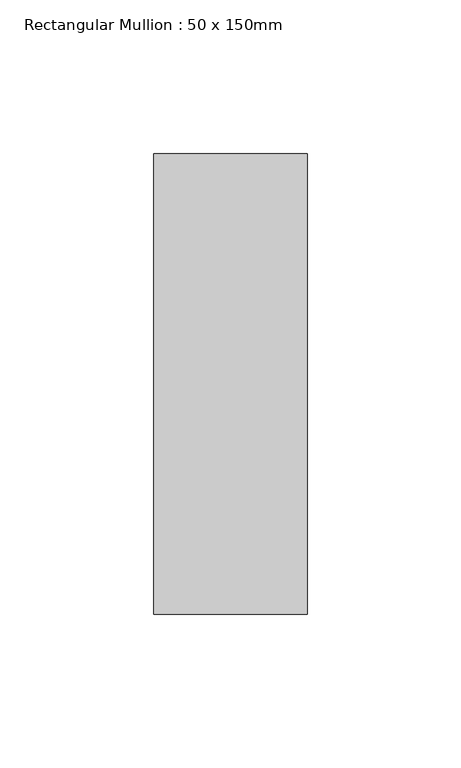
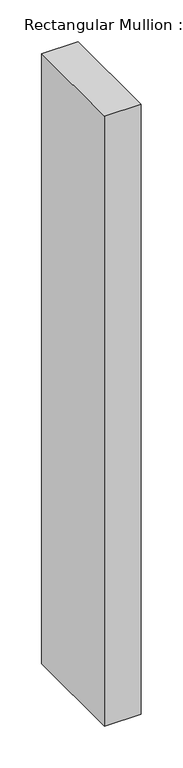
"""IFC4 building model written with IfcOpenShell, lengths in millimetres: member geometry, Rectangular Mullion : 50 x 150mm."""

import ifcopenshell
import ifcopenshell.guid

model = None  # the IFC model being written
_history = None  # IfcOwnerHistory: only IFC2X3 demands one
_inside = {}  # id of a spatial element -> (the spatial element, [elements in it])
_under = {}  # id of a project, library or spatial element -> (it, [spatial elements below it])
_declared = {}  # id of a project -> (the project, [libraries it declares])
_typed = {}  # id of a type object -> (the type object, [elements of that type])
_made_of = {}  # id of a material, layer set ... -> (it, [elements and type objects made of it])


def new_model(schema):
    """Start an empty IFC model of exactly this schema.

    Asked for "IFC4X3", IfcOpenShell would pick the latest addendum, in which some entities
    have other attributes; the version numbers below select the first issue.
    IFC2X3 requires an IfcOwnerHistory on every rooted entity: one is made here for all.
    """
    global model, _history
    if schema == "IFC4X3":
        model = ifcopenshell.file(schema_version=(4, 3, 0, 0))
    else:
        model = ifcopenshell.file(schema=schema)
    _inside.clear()
    _under.clear()
    _declared.clear()
    _typed.clear()
    _made_of.clear()
    _history = None
    if model.schema == "IFC2X3":
        org = make("IfcOrganization", Name="unknown")
        user = make(
            "IfcPersonAndOrganization",
            ThePerson=make("IfcPerson", FamilyName="unknown"),
            TheOrganization=org,
        )
        app = make(
            "IfcApplication",
            ApplicationDeveloper=org,
            Version="unknown",
            ApplicationFullName="unknown",
            ApplicationIdentifier="unknown",
        )
        _history = make(
            "IfcOwnerHistory",
            OwningUser=user,
            OwningApplication=app,
            ChangeAction="ADDED",
            CreationDate=0,
        )
    return model


def make(cls, **values):
    """One entity of the class cls with the attributes given. An attribute that is None is left unset."""
    return model.create_entity(
        cls, **{name: value for name, value in values.items() if value is not None}
    )


def rooted(cls, **values):
    """An entity with a GlobalId (a new one), such as an element, a storey or a relation."""
    return make(cls, GlobalId=ifcopenshell.guid.new(), OwnerHistory=_history, **values)


def si_unit(unit_type, name, prefix=None):
    """IfcSIUnit, for example si_unit("LENGTHUNIT", "METRE", prefix="MILLI")."""
    return make("IfcSIUnit", UnitType=unit_type, Prefix=prefix, Name=name)


def assignment(units):
    """IfcUnitAssignment: the units of a project."""
    return None if units is None else make("IfcUnitAssignment", Units=units)


def point(xyz):
    """IfcCartesianPoint."""
    return None if xyz is None else make("IfcCartesianPoint", Coordinates=xyz)


def direction(xyz):
    """IfcDirection."""
    return None if xyz is None else make("IfcDirection", DirectionRatios=xyz)


def frame(location, z_axis=None, x_axis=None):
    """IfcAxis2Placement3D, a coordinate frame: its origin and axes. An axis left out is left unset."""
    return make(
        "IfcAxis2Placement3D",
        Location=point(location),
        Axis=direction(z_axis),
        RefDirection=direction(x_axis),
    )


def origin():
    """The frame at (0, 0, 0) with its axes left unset."""
    return frame((0.0, 0.0, 0.0))


def place(relative_to, where):
    """IfcLocalPlacement: puts the frame where relative to a parent placement (None: the world)."""
    return make(
        "IfcLocalPlacement", PlacementRelTo=relative_to, RelativePlacement=where
    )


def context(
    kind, dimensions, precision=None, world=None, true_north=None, identifier=None
):
    """IfcGeometricRepresentationContext, for example the 3D "Model" context."""
    return make(
        "IfcGeometricRepresentationContext",
        ContextIdentifier=identifier,
        ContextType=kind,
        CoordinateSpaceDimension=dimensions,
        Precision=precision,
        WorldCoordinateSystem=world,
        TrueNorth=true_north,
    )


def project(units=None, contexts=None):
    """IfcProject with its units and contexts."""
    return rooted(
        "IfcProject",
        Name="project",
        RepresentationContexts=contexts,
        UnitsInContext=assignment(units),
    )


def spatial(cls, under=None, at=None, **own):
    """A site, building, storey or space (cls), placed at a placement, below another one or the project."""
    s = rooted(cls, ObjectPlacement=at, **own)
    if under is not None:
        _under.setdefault(under.id(), (under, []))[1].append(s)
    return s


def polyline(points):
    """IfcPolyline through the points."""
    return make("IfcPolyline", Points=[point(p) for p in points])


def outline(outer, holes=None, kind="AREA"):
    """IfcArbitraryClosedProfileDef: a profile drawn as a closed curve; with holes, ...WithVoids."""
    if holes is None:
        return make("IfcArbitraryClosedProfileDef", ProfileType=kind, OuterCurve=outer)
    return make(
        "IfcArbitraryProfileDefWithVoids",
        ProfileType=kind,
        OuterCurve=outer,
        InnerCurves=holes,
    )


def extrude(swept, where, along, depth):
    """IfcExtrudedAreaSolid: the profile swept, set in the frame where, extruded along a direction by depth."""
    return make(
        "IfcExtrudedAreaSolid",
        SweptArea=swept,
        Position=where,
        ExtrudedDirection=direction(along),
        Depth=depth,
    )


def shape(context_of_items, identifier, shape_type, items):
    """IfcShapeRepresentation: the items that make up one representation, for example the "Body"."""
    return make(
        "IfcShapeRepresentation",
        ContextOfItems=context_of_items,
        RepresentationIdentifier=identifier,
        RepresentationType=shape_type,
        Items=items,
    )


def source(mapping_origin, context_of_items, identifier, shape_type, items):
    """IfcRepresentationMap: a shape defined once, which mapped items show again and again."""
    return make(
        "IfcRepresentationMap",
        MappingOrigin=mapping_origin,
        MappedRepresentation=shape(context_of_items, identifier, shape_type, items),
    )


def transform(
    local_origin,
    x_axis=None,
    y_axis=None,
    z_axis=None,
    scale=None,
    scale2=None,
    scale3=None,
    uniform=True,
):
    """IfcCartesianTransformationOperator3D, or its non-uniform kind. x_axis, y_axis, z_axis: its Axis1, 2, 3."""
    if uniform:
        return make(
            "IfcCartesianTransformationOperator3D",
            Axis1=direction(x_axis),
            Axis2=direction(y_axis),
            LocalOrigin=point(local_origin),
            Scale=scale,
            Axis3=direction(z_axis),
        )
    return make(
        "IfcCartesianTransformationOperator3DnonUniform",
        Axis1=direction(x_axis),
        Axis2=direction(y_axis),
        LocalOrigin=point(local_origin),
        Scale=scale,
        Axis3=direction(z_axis),
        Scale2=scale2,
        Scale3=scale3,
    )


def mapped(mapping_source, mapping_target):
    """IfcMappedItem: shows the shape of a source again, moved by a transform."""
    return make(
        "IfcMappedItem", MappingSource=mapping_source, MappingTarget=mapping_target
    )


def made_of(thing, what):
    """Note that an element or type object is made of a material, layer set ...; save() writes the relation."""
    if what is not None:
        _made_of.setdefault(what.id(), (what, []))[1].append(thing)
    return thing


def element(
    cls,
    number,
    at=None,
    inside=None,
    cuts=None,
    type_object=None,
    material=None,
    context=None,
    identifier="Body",
    shape_type=None,
    held_by="IfcProductDefinitionShape",
    body=None,
    shapes=None,
    **own,
):
    """One element of the class cls, such as IfcWall. Its Tag is "e" and its number.

    at: its placement. inside: the storey or other place that contains it. cuts: it is an
    opening in that element (IfcRelVoidsElement). A single representation is given by context,
    identifier, shape_type and body (its items); several are given by shapes. held_by: the class
    of the entity that holds the representations. save() writes the other relations.
    """
    e = rooted(cls, Tag="e%d" % number, ObjectPlacement=at, **own)
    if body is not None:
        shapes = [shape(context, identifier, shape_type, body)]
    if shapes is not None:
        e.Representation = make(held_by, Representations=shapes)
    if inside is not None:
        _inside.setdefault(inside.id(), (inside, []))[1].append(e)
    if cuts is not None:
        rooted(
            "IfcRelVoidsElement", RelatingBuildingElement=cuts, RelatedOpeningElement=e
        )
    if type_object is not None:
        _typed.setdefault(type_object.id(), (type_object, []))[1].append(e)
    return made_of(e, material)


def aggregate(whole, parts):
    """IfcRelAggregates: a whole, such as a stair, and the parts it consists of."""
    return rooted("IfcRelAggregates", RelatingObject=whole, RelatedObjects=parts)


def save(model, path):
    """Write the relations noted so far, then the file.

    IfcRelAggregates (storeys below a building ...), IfcRelContainedInSpatialStructure (elements
    in a storey), IfcRelDefinesByType, IfcRelAssociatesMaterial and IfcRelDeclares: one each for
    every whole, place, type object, material and project.
    """
    for whole, parts in _under.values():
        aggregate(whole, parts)
    for where, things in _inside.values():
        rooted(
            "IfcRelContainedInSpatialStructure",
            RelatedElements=things,
            RelatingStructure=where,
        )
    for kind, things in _typed.values():
        rooted("IfcRelDefinesByType", RelatedObjects=things, RelatingType=kind)
    for what, things in _made_of.values():
        rooted("IfcRelAssociatesMaterial", RelatedObjects=things, RelatingMaterial=what)
    for by, libraries in _declared.values():
        rooted("IfcRelDeclares", RelatingContext=by, RelatedDefinitions=libraries)
    model.write(path)


def rectangular_mullion_50_x_150mm_6e645c27(model_context):
    return source(origin(), model_context, "Body", "SweptSolid", [
        extrude(outline(polyline([(25.0, 75.0), (25.0, -75.0), (-25.0, -75.0), (-25.0, 75.0), (25.0, 75.0)])), frame((0.0, 0.0, -887.5), z_axis=(0.0, 0.0, 1.0), x_axis=(1.0, 0.0, 0.0)), (0.0, 0.0, 1.0), 887.5),
    ])


if __name__ == "__main__":
    model = new_model("IFC4")
    model_context = context("Model", 3, world=origin())
    ifc_project = project(units=[si_unit("LENGTHUNIT", "METRE", prefix="MILLI")], contexts=[model_context])
    site = spatial("IfcSite", under=ifc_project)
    building = spatial("IfcBuilding", under=site)
    placement = place(None, origin())
    rectangular_mullion_50_x_150mm_shape = rectangular_mullion_50_x_150mm_6e645c27(model_context)
    element("IfcMember", 1, ObjectType="Rectangular Mullion : 50 x 150mm", at=placement, inside=building, context=model_context, shape_type="MappedRepresentation", body=[
        mapped(rectangular_mullion_50_x_150mm_shape, transform((0.0, 0.0, 0.0), x_axis=(1.0, 0.0, 0.0), y_axis=(0.0, 1.0, 0.0), z_axis=(0.0, 0.0, 1.0))),
    ])
    save(model, "model.ifc")

# Revit data of these elements
# Type "Rectangular Mullion : 50 x 150mm"
#   built-in parameter 1007304 = 0.492126 (stored number, unit not read)
#   built-in parameter 1007301 = 0.082021 (stored number, unit not read)
#   built-in parameter 1007300 = 0.082021 (stored number, unit not read)
# Element 1 (IfcMember, "Rectangular Mullion : 50 x 150mm")
#   Materials on its faces: "Aluminium"
# Materials
#   "Aluminium": class "Metal", colour RGB 247 247 247, transparency 0, Description = "Aluminium 6061", Cost = 0
